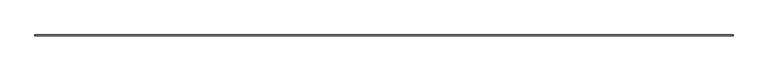
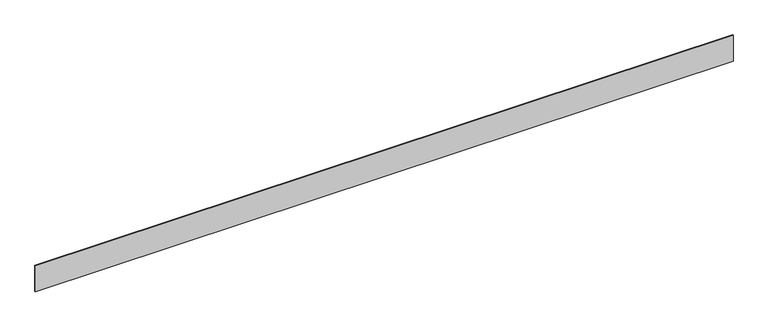
"""IFC4 building model written with IfcOpenShell, lengths in millimetres: proxy geometry, Generic Models 6:Generic Models 2:318829:Generic Models 2:318829 : Generic Models 6:Generic Models 2:318829:19 : Generic Models 6:Generic Models 2:318829:Generic Models 2:318829 : Generic Models 6:Generic Models 2:318829:300683."""

from ifc_helpers import new_model, si_unit, origin, origin_with_axes, place, context, project, spatial, polyline, outline, extrude, source, transform, mapped, element, save


def generic_models_7b58e61b(model_context):
    return source(origin(), model_context, "Body", "SweptSolid", [
        extrude(outline(polyline([(592758.9138536, -579025.918279), (592758.9138536, -579029.093279), (590317.0242239, -579029.093279), (590317.0242239, -579025.918279), (592758.9138536, -579025.918279)])), origin_with_axes(), (0.0, 0.0, 1.0), 95.25),
    ])


if __name__ == "__main__":
    model = new_model("IFC4")
    model_context = context("Model", 3, world=origin())
    ifc_project = project(units=[si_unit("LENGTHUNIT", "METRE", prefix="MILLI")], contexts=[model_context])
    site = spatial("IfcSite", under=ifc_project)
    building = spatial("IfcBuilding", under=site)
    placement = place(None, origin())
    generic_models_shape = generic_models_7b58e61b(model_context)
    element("IfcBuildingElementProxy", 1, Name="Generic Models 6:Generic Models 2:318829:Generic Models 2:318829 : Generic Models 6:Generic Models 2:318829:19 : Generic Models 6:Generic Models 2:318829:Generic Models 2:318829 : Generic Models 6:Generic Models 2:318829:300683", ObjectType="Generic Models 6:Generic Models 2:318829:Generic Models 2:318829 : Generic Models 6:Generic Models 2:318829:19 : Generic Models 6:Generic Models 2:318829:Generic Models 2:318829 : Generic Models 6:Generic Models 2:318829:300683", at=placement, inside=building, context=model_context, shape_type="MappedRepresentation", body=[
        mapped(generic_models_shape, transform((0.0, 0.0, 0.0), x_axis=(1.0, 0.0, 0.0), y_axis=(0.0, 1.0, 0.0), z_axis=(0.0, 0.0, 1.0))),
    ])
    save(model, "model.ifc")

# Revit data of these elements
# Type "Generic Models 6:Generic Models 2:318829:Generic Models 2:318829 : Generic Models 6:Generic Models 2:318829:19 : Generic Models 6:Generic Models 2:318829:Generic Models 2:318829 : Generic Models 6:Generic Models 2:318829:300683"
#   NameOverride = "Generic Models 6:Generic Models 2:318829:Generic Models 2:318829 : Generic Models 6:Generic Models 2:318829:300683"
#   ObjectTypeOverride = "Generic Models 2:318829 : Generic Models 6:Generic Models 2:318829"
#   Reference = "Generic Models 2"
#   Tag = "300683"
# Element 1 (IfcBuildingElementProxy, "Generic Models 6:Generic Models 2:318829:Generic Models 2:318829 : Generic Models 6:Generic Models 2:318829:19 : Generic Models 6:Generic Models 2:318829:Generic Models 2:318829 : Generic Models 6:Generic Models 2:318829:300683")
#   Materials on its faces: "ALUM. BASE TRIM"
# Materials
#   "ALUM. BASE TRIM": class "Generic", colour RGB 120 120 120, transparency 0, Cost = 0
